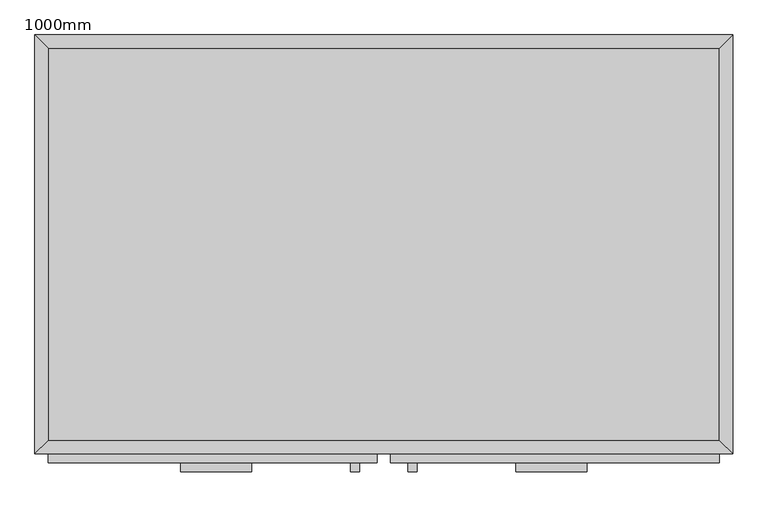
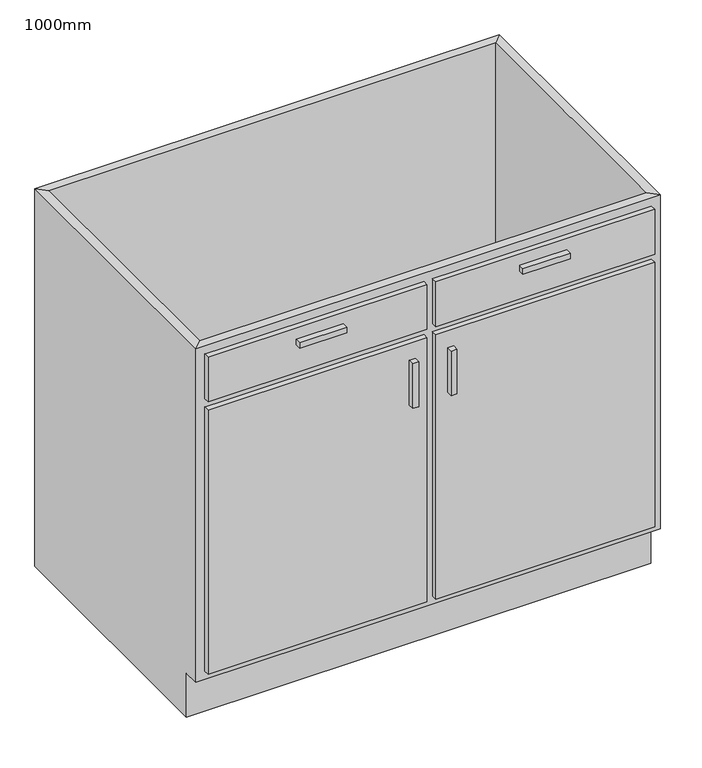
"""IFC4 building model written with IfcOpenShell, lengths in millimetres: furniture geometry, M_Base Cabinet-Double Door & 2 Drawer : 1000mm."""

import ifcopenshell
import ifcopenshell.guid

model = None  # the IFC model being written
_history = None  # IfcOwnerHistory: only IFC2X3 demands one
_inside = {}  # id of a spatial element -> (the spatial element, [elements in it])
_under = {}  # id of a project, library or spatial element -> (it, [spatial elements below it])
_declared = {}  # id of a project -> (the project, [libraries it declares])
_typed = {}  # id of a type object -> (the type object, [elements of that type])
_made_of = {}  # id of a material, layer set ... -> (it, [elements and type objects made of it])


def new_model(schema):
    """Start an empty IFC model of exactly this schema.

    Asked for "IFC4X3", IfcOpenShell would pick the latest addendum, in which some entities
    have other attributes; the version numbers below select the first issue.
    IFC2X3 requires an IfcOwnerHistory on every rooted entity: one is made here for all.
    """
    global model, _history
    if schema == "IFC4X3":
        model = ifcopenshell.file(schema_version=(4, 3, 0, 0))
    else:
        model = ifcopenshell.file(schema=schema)
    _inside.clear()
    _under.clear()
    _declared.clear()
    _typed.clear()
    _made_of.clear()
    _history = None
    if model.schema == "IFC2X3":
        org = make("IfcOrganization", Name="unknown")
        user = make(
            "IfcPersonAndOrganization",
            ThePerson=make("IfcPerson", FamilyName="unknown"),
            TheOrganization=org,
        )
        app = make(
            "IfcApplication",
            ApplicationDeveloper=org,
            Version="unknown",
            ApplicationFullName="unknown",
            ApplicationIdentifier="unknown",
        )
        _history = make(
            "IfcOwnerHistory",
            OwningUser=user,
            OwningApplication=app,
            ChangeAction="ADDED",
            CreationDate=0,
        )
    return model


def make(cls, **values):
    """One entity of the class cls with the attributes given. An attribute that is None is left unset."""
    return model.create_entity(
        cls, **{name: value for name, value in values.items() if value is not None}
    )


def rooted(cls, **values):
    """An entity with a GlobalId (a new one), such as an element, a storey or a relation."""
    return make(cls, GlobalId=ifcopenshell.guid.new(), OwnerHistory=_history, **values)


def si_unit(unit_type, name, prefix=None):
    """IfcSIUnit, for example si_unit("LENGTHUNIT", "METRE", prefix="MILLI")."""
    return make("IfcSIUnit", UnitType=unit_type, Prefix=prefix, Name=name)


def assignment(units):
    """IfcUnitAssignment: the units of a project."""
    return None if units is None else make("IfcUnitAssignment", Units=units)


def point(xyz):
    """IfcCartesianPoint."""
    return None if xyz is None else make("IfcCartesianPoint", Coordinates=xyz)


def direction(xyz):
    """IfcDirection."""
    return None if xyz is None else make("IfcDirection", DirectionRatios=xyz)


def frame(location, z_axis=None, x_axis=None):
    """IfcAxis2Placement3D, a coordinate frame: its origin and axes. An axis left out is left unset."""
    return make(
        "IfcAxis2Placement3D",
        Location=point(location),
        Axis=direction(z_axis),
        RefDirection=direction(x_axis),
    )


def origin():
    """The frame at (0, 0, 0) with its axes left unset."""
    return frame((0.0, 0.0, 0.0))


def place(relative_to, where):
    """IfcLocalPlacement: puts the frame where relative to a parent placement (None: the world)."""
    return make(
        "IfcLocalPlacement", PlacementRelTo=relative_to, RelativePlacement=where
    )


def context(
    kind, dimensions, precision=None, world=None, true_north=None, identifier=None
):
    """IfcGeometricRepresentationContext, for example the 3D "Model" context."""
    return make(
        "IfcGeometricRepresentationContext",
        ContextIdentifier=identifier,
        ContextType=kind,
        CoordinateSpaceDimension=dimensions,
        Precision=precision,
        WorldCoordinateSystem=world,
        TrueNorth=true_north,
    )


def project(units=None, contexts=None):
    """IfcProject with its units and contexts."""
    return rooted(
        "IfcProject",
        Name="project",
        RepresentationContexts=contexts,
        UnitsInContext=assignment(units),
    )


def spatial(cls, under=None, at=None, **own):
    """A site, building, storey or space (cls), placed at a placement, below another one or the project."""
    s = rooted(cls, ObjectPlacement=at, **own)
    if under is not None:
        _under.setdefault(under.id(), (under, []))[1].append(s)
    return s


def polyline(points):
    """IfcPolyline through the points."""
    return make("IfcPolyline", Points=[point(p) for p in points])


def outline(outer, holes=None, kind="AREA"):
    """IfcArbitraryClosedProfileDef: a profile drawn as a closed curve; with holes, ...WithVoids."""
    if holes is None:
        return make("IfcArbitraryClosedProfileDef", ProfileType=kind, OuterCurve=outer)
    return make(
        "IfcArbitraryProfileDefWithVoids",
        ProfileType=kind,
        OuterCurve=outer,
        InnerCurves=holes,
    )


def extrude(swept, where, along, depth):
    """IfcExtrudedAreaSolid: the profile swept, set in the frame where, extruded along a direction by depth."""
    return make(
        "IfcExtrudedAreaSolid",
        SweptArea=swept,
        Position=where,
        ExtrudedDirection=direction(along),
        Depth=depth,
    )


def faces_of(points, faces, orient=None, outer=None):
    """IfcFace entities. A face is a list of loops; a loop is a list of indices into points, from 0.

    orient and outer hold one flag for each loop. By default every Orientation is true, the
    first loop of a face is its IfcFaceOuterBound and the others are IfcFaceBound.
    """
    made = []
    for i, loops in enumerate(faces):
        bounds = []
        for j, loop in enumerate(loops):
            is_outer = j == 0 if outer is None else outer[i][j]
            bounds.append(
                make(
                    "IfcFaceOuterBound" if is_outer else "IfcFaceBound",
                    Bound=make("IfcPolyLoop", Polygon=[points[k] for k in loop]),
                    Orientation=True if orient is None else orient[i][j],
                )
            )
        made.append(make("IfcFace", Bounds=bounds))
    return made


def faceted_brep(points, faces, orient=None, outer=None, voids=None):
    """IfcFacetedBrep: a solid bounded by flat faces; with voids (closed shells), ...WithVoids."""
    shared = [point(p) for p in points]
    hull = make("IfcClosedShell", CfsFaces=faces_of(shared, faces, orient, outer))
    if voids is None:
        return make("IfcFacetedBrep", Outer=hull)
    return make(
        "IfcFacetedBrepWithVoids",
        Outer=hull,
        Voids=[
            make(cls, CfsFaces=faces_of(shared, fs, o, b)) for cls, fs, o, b in voids
        ],
    )


def shape(context_of_items, identifier, shape_type, items):
    """IfcShapeRepresentation: the items that make up one representation, for example the "Body"."""
    return make(
        "IfcShapeRepresentation",
        ContextOfItems=context_of_items,
        RepresentationIdentifier=identifier,
        RepresentationType=shape_type,
        Items=items,
    )


def source(mapping_origin, context_of_items, identifier, shape_type, items):
    """IfcRepresentationMap: a shape defined once, which mapped items show again and again."""
    return make(
        "IfcRepresentationMap",
        MappingOrigin=mapping_origin,
        MappedRepresentation=shape(context_of_items, identifier, shape_type, items),
    )


def transform(
    local_origin,
    x_axis=None,
    y_axis=None,
    z_axis=None,
    scale=None,
    scale2=None,
    scale3=None,
    uniform=True,
):
    """IfcCartesianTransformationOperator3D, or its non-uniform kind. x_axis, y_axis, z_axis: its Axis1, 2, 3."""
    if uniform:
        return make(
            "IfcCartesianTransformationOperator3D",
            Axis1=direction(x_axis),
            Axis2=direction(y_axis),
            LocalOrigin=point(local_origin),
            Scale=scale,
            Axis3=direction(z_axis),
        )
    return make(
        "IfcCartesianTransformationOperator3DnonUniform",
        Axis1=direction(x_axis),
        Axis2=direction(y_axis),
        LocalOrigin=point(local_origin),
        Scale=scale,
        Axis3=direction(z_axis),
        Scale2=scale2,
        Scale3=scale3,
    )


def mapped(mapping_source, mapping_target):
    """IfcMappedItem: shows the shape of a source again, moved by a transform."""
    return make(
        "IfcMappedItem", MappingSource=mapping_source, MappingTarget=mapping_target
    )


def made_of(thing, what):
    """Note that an element or type object is made of a material, layer set ...; save() writes the relation."""
    if what is not None:
        _made_of.setdefault(what.id(), (what, []))[1].append(thing)
    return thing


def element(
    cls,
    number,
    at=None,
    inside=None,
    cuts=None,
    type_object=None,
    material=None,
    context=None,
    identifier="Body",
    shape_type=None,
    held_by="IfcProductDefinitionShape",
    body=None,
    shapes=None,
    **own,
):
    """One element of the class cls, such as IfcWall. Its Tag is "e" and its number.

    at: its placement. inside: the storey or other place that contains it. cuts: it is an
    opening in that element (IfcRelVoidsElement). A single representation is given by context,
    identifier, shape_type and body (its items); several are given by shapes. held_by: the class
    of the entity that holds the representations. save() writes the other relations.
    """
    e = rooted(cls, Tag="e%d" % number, ObjectPlacement=at, **own)
    if body is not None:
        shapes = [shape(context, identifier, shape_type, body)]
    if shapes is not None:
        e.Representation = make(held_by, Representations=shapes)
    if inside is not None:
        _inside.setdefault(inside.id(), (inside, []))[1].append(e)
    if cuts is not None:
        rooted(
            "IfcRelVoidsElement", RelatingBuildingElement=cuts, RelatedOpeningElement=e
        )
    if type_object is not None:
        _typed.setdefault(type_object.id(), (type_object, []))[1].append(e)
    return made_of(e, material)


def aggregate(whole, parts):
    """IfcRelAggregates: a whole, such as a stair, and the parts it consists of."""
    return rooted("IfcRelAggregates", RelatingObject=whole, RelatedObjects=parts)


def save(model, path):
    """Write the relations noted so far, then the file.

    IfcRelAggregates (storeys below a building ...), IfcRelContainedInSpatialStructure (elements
    in a storey), IfcRelDefinesByType, IfcRelAssociatesMaterial and IfcRelDeclares: one each for
    every whole, place, type object, material and project.
    """
    for whole, parts in _under.values():
        aggregate(whole, parts)
    for where, things in _inside.values():
        rooted(
            "IfcRelContainedInSpatialStructure",
            RelatedElements=things,
            RelatingStructure=where,
        )
    for kind, things in _typed.values():
        rooted("IfcRelDefinesByType", RelatedObjects=things, RelatingType=kind)
    for what, things in _made_of.values():
        rooted("IfcRelAssociatesMaterial", RelatedObjects=things, RelatingMaterial=what)
    for by, libraries in _declared.values():
        rooted("IfcRelDeclares", RelatingContext=by, RelatedDefinitions=libraries)
    model.write(path)


def furniture_1000mm_952fdc5e(model_context):
    return source(origin(), model_context, "Body", "SolidModel", [
        faceted_brep([(499.6877049, -580.95, 860.0), (499.6877049, -580.95, 100.0), (-462.2122951, -580.95, 100.0), (-462.2122951, -580.95, 860.0), (-481.2622951, -600.0, 860.0), (518.7377049, -600.0, 860.0), (-481.2622951, -600.0, 100.0), (518.7377049, -600.0, 100.0), (-462.2122951, -565.0, 100.0), (-462.2122951, -19.05, 100.0), (-462.2122951, -19.05, 860.0), (-481.2622951, 0.0, 860.0), (-481.2622951, 0.0, 0.0), (-481.2622951, -565.0, 0.0), (-481.2622951, -565.0, 100.0), (499.6877049, -19.05, 100.0), (499.6877049, -19.05, 860.0), (518.7377049, 0.0, 860.0), (518.7377049, 0.0, 0.0), (499.6877049, -565.0, 100.0), (518.7377049, -565.0, 100.0), (518.7377049, -565.0, 0.0)], [[[0, 1, 2, 3]], [[0, 3, 4, 5]], [[5, 4, 6, 7]], [[2, 1, 7, 6]], [[3, 2, 8, 9, 10]], [[4, 3, 10, 11]], [[6, 4, 11, 12, 13, 14]], [[2, 6, 14, 8]], [[10, 9, 15, 16]], [[11, 10, 16, 17]], [[12, 11, 17, 18]], [[1, 0, 16, 15, 19]], [[0, 5, 17, 16]], [[5, 7, 20, 21, 18, 17]], [[7, 1, 19, 20]], [[8, 19, 15, 9]], [[18, 21, 13, 12]], [[13, 21, 20, 19, 8, 14]]]),
        extrude(outline(polyline([(-170.9372951, -625.4), (-272.5372951, -625.4), (-272.5372951, -612.7), (-170.9372951, -612.7), (-170.9372951, -625.4)])), frame((0.0, 0.0, 802.85), z_axis=(0.0, 0.0, 1.0), x_axis=(1.0, 0.0, 0.0)), (0.0, 0.0, 1.0), 12.7),
        extrude(outline(polyline([(310.0127049, -625.4), (208.4127049, -625.4), (208.4127049, -612.7), (310.0127049, -612.7), (310.0127049, -625.4)])), frame((0.0, 0.0, 802.85), z_axis=(0.0, 0.0, 1.0), x_axis=(1.0, 0.0, 0.0)), (0.0, 0.0, 1.0), 12.7),
        extrude(outline(polyline([(-16.1872951, -625.4), (-28.8872951, -625.4), (-28.8872951, -612.7), (-16.1872951, -612.7), (-16.1872951, -625.4)])), frame((0.0, 0.0, 580.6), z_axis=(0.0, 0.0, 1.0), x_axis=(1.0, 0.0, 0.0)), (0.0, 0.0, 1.0), 101.6),
        extrude(outline(polyline([(66.3627049, -625.4), (53.6627049, -625.4), (53.6627049, -612.7), (66.3627049, -612.7), (66.3627049, -625.4)])), frame((0.0, 0.0, 580.6), z_axis=(0.0, 0.0, 1.0), x_axis=(1.0, 0.0, 0.0)), (0.0, 0.0, 1.0), 101.6),
        extrude(outline(polyline([(9.2127049, -612.7), (-462.2122951, -612.7), (-462.2122951, -600.0), (9.2127049, -600.0), (9.2127049, -612.7)])), frame((0.0, 0.0, 739.35), z_axis=(0.0, 0.0, 1.0), x_axis=(1.0, 0.0, 0.0)), (0.0, 0.0, 1.0), 101.6),
        extrude(outline(polyline([(499.6877049, -612.7), (28.2627049, -612.7), (28.2627049, -600.0), (499.6877049, -600.0), (499.6877049, -612.7)])), frame((0.0, 0.0, 739.35), z_axis=(0.0, 0.0, 1.0), x_axis=(1.0, 0.0, 0.0)), (0.0, 0.0, 1.0), 101.6),
        extrude(outline(polyline([(9.2127049, -612.7), (-462.2122951, -612.7), (-462.2122951, -600.0), (9.2127049, -600.0), (9.2127049, -612.7)])), frame((0.0, 0.0, 119.05), z_axis=(0.0, 0.0, 1.0), x_axis=(1.0, 0.0, 0.0)), (0.0, 0.0, 1.0), 601.25),
        extrude(outline(polyline([(499.6877049, -612.7), (28.2627049, -612.7), (28.2627049, -600.0), (499.6877049, -600.0), (499.6877049, -612.7)])), frame((0.0, 0.0, 119.05), z_axis=(0.0, 0.0, 1.0), x_axis=(1.0, 0.0, 0.0)), (0.0, 0.0, 1.0), 601.25),
        extrude(outline(polyline([(499.6877049, -19.05), (499.6877049, -580.95), (-462.2122951, -580.95), (-462.2122951, -19.05), (499.6877049, -19.05)])), frame((0.0, 0.0, 100.0), z_axis=(0.0, 0.0, 1.0), x_axis=(1.0, 0.0, 0.0)), (0.0, 0.0, 1.0), 19.05),
    ])


if __name__ == "__main__":
    model = new_model("IFC4")
    model_context = context("Model", 3, world=origin())
    ifc_project = project(units=[si_unit("LENGTHUNIT", "METRE", prefix="MILLI")], contexts=[model_context])
    site = spatial("IfcSite", under=ifc_project)
    building = spatial("IfcBuilding", under=site)
    placement = place(None, origin())
    furniture_1000mm_shape = furniture_1000mm_952fdc5e(model_context)
    element("IfcFurniture", 1, ObjectType="M_Base Cabinet-Double Door & 2 Drawer : 1000mm", at=placement, inside=building, context=model_context, shape_type="MappedRepresentation", body=[
        mapped(furniture_1000mm_shape, transform((0.0, 0.0, 0.0), x_axis=(1.0, 0.0, 0.0), y_axis=(0.0, 1.0, 0.0), z_axis=(0.0, 0.0, 1.0))),
    ])
    save(model, "model.ifc")

# Revit data of these elements
# Type "M_Base Cabinet-Double Door & 2 Drawer : 1000mm"
#   Manufacturer = "Manufacturer"
#   Finish = "Finish"
#   Construction Type = "Construction Type"
#   AccessibilityPerformance = "AccessibilityPerformance"
#   CodePerformance = "CodePerformance"
#   Area = "Area"
#   Color = "Color"
#   Constituents = "Constituents"
#   Features = "Features"
#   Finish = "Finish"
#   Grade = "Grade"
#   Material = "Material"
#   ModelReference = "ModelReference"
#   NominalHeight = "NominalHeight"
#   NominalLength = "NominalLength"
#   NominalWidth = "NominalWidth"
#   ProductionYear = "ProductionYear"
#   Reference = "Reference"
#   Shape = "Shape"
#   Size = "Size"
#   SustainabilityPerformance = "SustainabilityPerformance"
#   WarrantyDescription = "WarrantyDescription"
#   WarrantyDurationLabor = "WarrantyDurationLabor"
#   WarrantyDurationParts = "WarrantyDurationParts"
#   WarrantyGuarantorLabor = "WarrantyGuarantorLabor"
#   WarrantyGuarantorParts = "WarrantyGuarantorParts"
#   ExpectedLife = "ExpectedLife"
#   ReplacementCost = "ReplacementCost"
#   AssetAccountingType = "FIXED"
#   ModelLabel = "ModelLabel"
#   Depth = 0.600 m
#   Height = 0.860 m
#   Plinth Depth = 0.035 m
#   Plinth Height = 0.100 m
#   Width = 1.000 m
#   Cabinet Material = none
#   Door/Drawer Material = none
#   Handle Material = Cabinets - Handles
# Element 1 (IfcFurniture, "M_Base Cabinet-Double Door & 2 Drawer : 1000mm")
#   Materials on its faces: "Cabinets", "Cabinets - Handles"
# Materials
#   "Cabinets - Handles": class "Metal", colour RGB 57 57 57, transparency 0
#   "Cabinets": class "Miscellaneous", colour RGB 249 249 249, transparency 0
